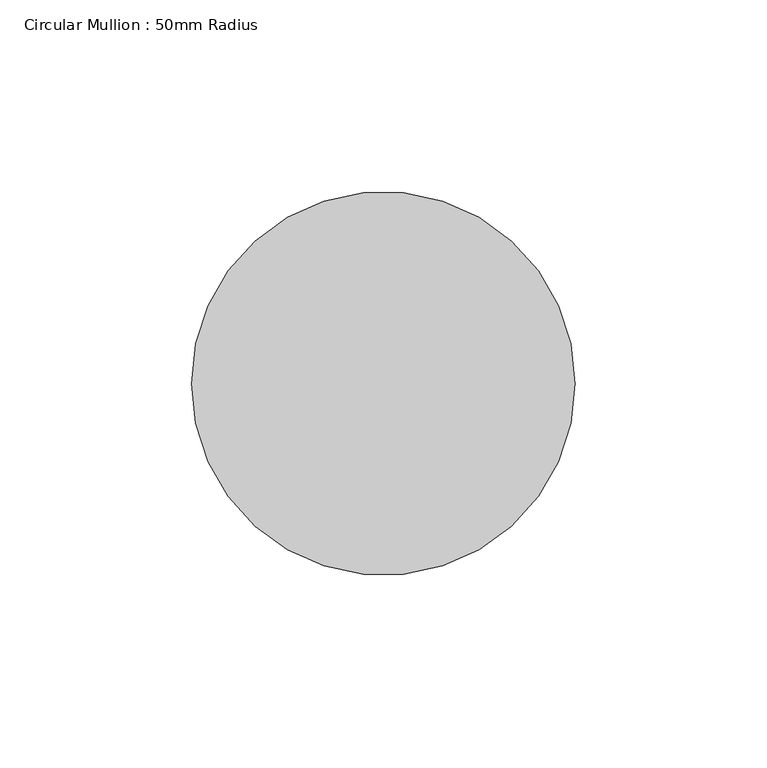
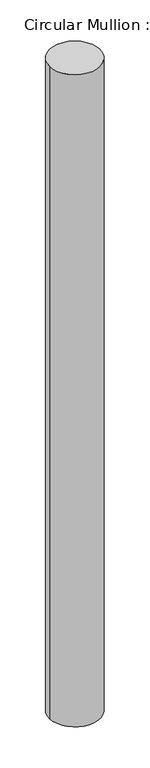
"""IFC4 building model written with IfcOpenShell, lengths in millimetres: member geometry, Circular Mullion : 50mm Radius."""

from ifc_helpers import new_model, si_unit, point, frame, origin, origin_2d, place, context, project, spatial, circle_curve, trimmed, segment, composite_curve, outline, extrude, source, transform, mapped, element, save


def circular_mullion_50mm_radius_dc060d00(model_context):
    return source(origin(), model_context, "Body", "SweptSolid", [
        extrude(outline(composite_curve([segment(trimmed(circle_curve(origin_2d(), 50.0), [point((50.0, 0.0))], [point((-50.0, 0.0))], False, "CARTESIAN"), True, "CONTINUOUS"), segment(trimmed(circle_curve(origin_2d(), 50.0), [point((-50.0, 0.0))], [point((50.0, 0.0))], False, "CARTESIAN"), True, "CONTINUOUS")], self_intersect=False)), frame((0.0, 0.0, -1355.9142183), z_axis=(0.0, 0.0, 1.0), x_axis=(1.0, 0.0, 0.0)), (0.0, 0.0, 1.0), 1355.9142183),
    ])


if __name__ == "__main__":
    model = new_model("IFC4")
    model_context = context("Model", 3, world=origin())
    ifc_project = project(units=[si_unit("LENGTHUNIT", "METRE", prefix="MILLI")], contexts=[model_context])
    site = spatial("IfcSite", under=ifc_project)
    building = spatial("IfcBuilding", under=site)
    placement = place(None, origin())
    circular_mullion_50mm_radius_shape = circular_mullion_50mm_radius_dc060d00(model_context)
    element("IfcMember", 1, ObjectType="Circular Mullion : 50mm Radius", at=placement, inside=building, context=model_context, shape_type="MappedRepresentation", body=[
        mapped(circular_mullion_50mm_radius_shape, transform((0.0, 0.0, 0.0), x_axis=(1.0, 0.0, 0.0), y_axis=(0.0, 1.0, 0.0), z_axis=(0.0, 0.0, 1.0))),
    ])
    save(model, "model.ifc")

# Revit data of these elements
# Type "Circular Mullion : 50mm Radius"
#   built-in parameter 1007350 = 0.164042 (stored number, unit not read)
# Element 1 (IfcMember, "Circular Mullion : 50mm Radius")
#   Materials on its faces: "Aluminium"
# Materials
#   "Aluminium": class "Metal", colour RGB 247 247 247, transparency 0, Description = "Aluminium 6061", Cost = 0
